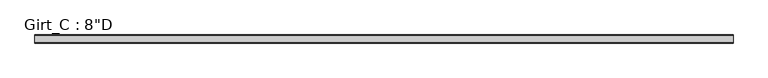
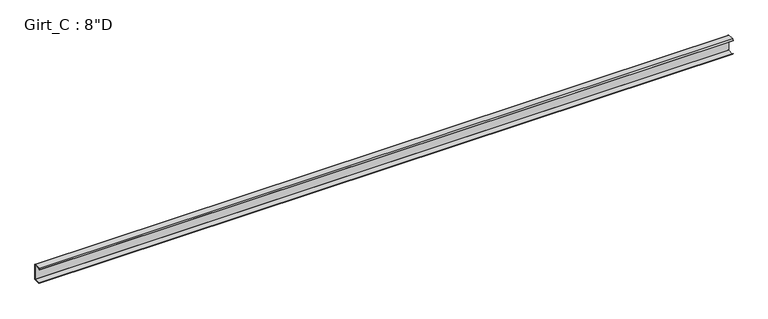
"""IFC4 building model written with IfcOpenShell, lengths in millimetres: beam geometry."""

from ifc_helpers import new_model, si_unit, point, frame, frame_2d, origin, place, context, project, spatial, polyline, circle_curve, trimmed, segment, composite_curve, outline, extrude, source, transform, mapped, element, save


def beam_b1523349(model_context):
    return source(origin(), model_context, "Body", "SweptSolid", [
        extrude(outline(composite_curve([segment(polyline([(-87.5109375, 101.6), (-3.3734375, 101.6)]), True, "CONTINUOUS"), segment(trimmed(circle_curve(frame_2d((-3.3734375, 96.8375)), 4.7625), [point((-3.3734375, 101.6))], [point((1.3890625, 96.8375))], False, "CARTESIAN"), True, "CONTINUOUS"), segment(polyline([(1.3890625, 96.8375), (1.3890625, -96.8375)]), True, "CONTINUOUS"), segment(trimmed(circle_curve(frame_2d((-3.3734375, -96.8375)), 4.7625), [point((1.3890625, -96.8375))], [point((-3.3734375, -101.6))], False, "CARTESIAN"), True, "CONTINUOUS"), segment(polyline([(-3.3734375, -101.6), (-87.5109375, -101.6), (-99.7792647, -86.979177), (-97.6510975, -85.1934327), (-86.2154765, -98.821875), (-3.2694106, -98.821875)]), True, "CONTINUOUS"), segment(trimmed(circle_curve(frame_2d((-3.3748024, -96.8389339)), 1.9857399), [point((-3.2694106, -98.821875))], [point((-1.3890625, -96.8389339))], True, "CARTESIAN"), True, "CONTINUOUS"), segment(polyline([(-1.3890625, -96.8389339), (-1.3890625, 96.8381931)]), True, "CONTINUOUS"), segment(trimmed(circle_curve(frame_2d((-3.3741066, 96.8381931)), 1.9850441), [point((-1.3890625, 96.8381931))], [point((-3.3005807, 98.821875))], True, "CARTESIAN"), True, "CONTINUOUS"), segment(polyline([(-3.3005807, 98.821875), (-86.2154765, 98.821875), (-97.6278742, 85.221109), (-99.7560415, 87.0068534), (-87.5109375, 101.6)]), True, "CONTINUOUS")], self_intersect=False)), frame((-4273.1678625, 0.0, 0.0), z_axis=(1.0, 0.0, 0.0), x_axis=(0.0, 1.0, 0.0)), (0.0, 0.0, 1.0), 8680.9330799),
    ])


if __name__ == "__main__":
    model = new_model("IFC4")
    model_context = context("Model", 3, world=origin())
    ifc_project = project(units=[si_unit("LENGTHUNIT", "METRE", prefix="MILLI")], contexts=[model_context])
    site = spatial("IfcSite", under=ifc_project)
    building = spatial("IfcBuilding", under=site)
    placement = place(None, origin())
    beam_shape = beam_b1523349(model_context)
    element("IfcBeam", 1, ObjectType="Girt_C : 8\"D", at=placement, inside=building, context=model_context, shape_type="MappedRepresentation", body=[
        mapped(beam_shape, transform((0.0, 0.0, 0.0), x_axis=(1.0, 0.0, 0.0), y_axis=(0.0, 1.0, 0.0), z_axis=(0.0, 0.0, 1.0))),
    ])
    save(model, "model.ifc")

# Revit data of these elements
# Type "Girt_C : 8\"D"
#   half leg = 0' - 1 3/4"
#   Web_Thickness = 0' - 0 7/64"
#   Length [instance default] = 10' - 0"
#   Leg_1 = 0' - 3 1/2"
#   Height = 0' - 8"
#   Structural Material [instance default] = none
# Element 1 (IfcBeam, "Girt_C : 8\"D")
#   Structural Material = GALVANIZED 'CEE' SECTION (8.0x3.5C - SEE STRUCT. DWGS)
#   Materials on its faces: "GALVANIZED 'CEE' SECTION (8.0x3.5C - SEE STRUCT. DWGS)"
# Materials
#   "GALVANIZED 'CEE' SECTION (8.0x3.5C - SEE STRUCT. DWGS)": class "Metal", colour RGB 137 146 153, transparency 0, Description = "Steel, mill finish", Cost = 0
